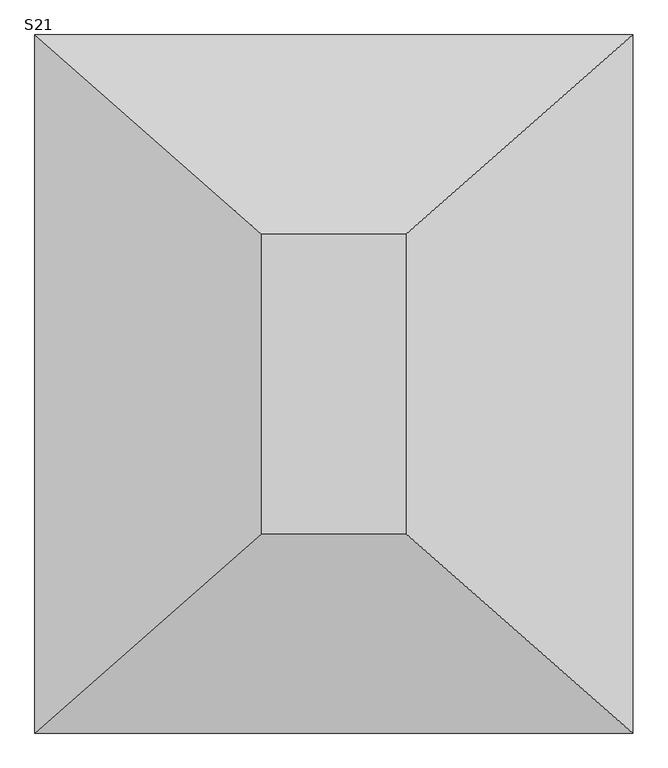
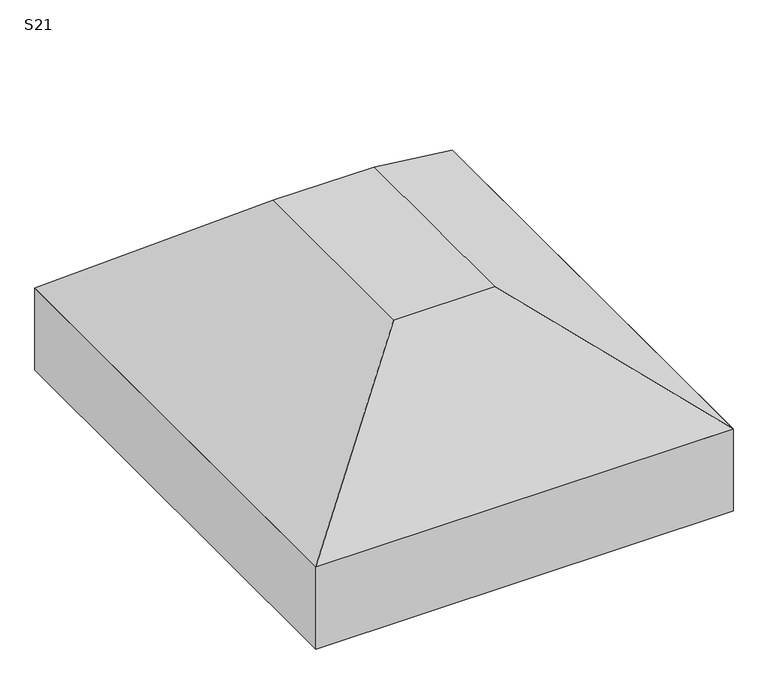
"""IFC4 building model written with IfcOpenShell, lengths in millimetres: fastener geometry, TQS - Sapata : S21."""

from ifc_helpers import new_model, si_unit, frame, origin, place, context, project, spatial, polyline, outline, extrude, faceted_brep, source, transform, mapped, element, save


def s21_dbbb6426(model_context):
    return source(origin(), model_context, "Body", "SolidModel", [
        faceted_brep([(-55.0, 100.0, 0.0), (-345.0, 100.0, 0.0), (-345.0, -500.0, 0.0), (-55.0, -500.0, 0.0), (400.0, 500.0, -350.0), (400.0, -900.0, -350.0), (-800.0, -900.0, -350.0), (-800.0, 500.0, -350.0)], [[[0, 1, 2, 3]], [[4, 5, 6, 7]], [[4, 7, 1, 0]], [[7, 6, 2, 1]], [[6, 5, 3, 2]], [[5, 4, 0, 3]]]),
        extrude(outline(polyline([(400.0, 500.0), (400.0, -900.0), (-800.0, -900.0), (-800.0, 500.0), (400.0, 500.0)])), frame((0.0, 0.0, -600.0), z_axis=(0.0, 0.0, 1.0), x_axis=(1.0, 0.0, 0.0)), (0.0, 0.0, 1.0), 250.0),
    ])


if __name__ == "__main__":
    model = new_model("IFC4")
    model_context = context("Model", 3, world=origin())
    ifc_project = project(units=[si_unit("LENGTHUNIT", "METRE", prefix="MILLI")], contexts=[model_context])
    site = spatial("IfcSite", under=ifc_project)
    building = spatial("IfcBuilding", under=site)
    placement = place(None, origin())
    s21_shape = s21_dbbb6426(model_context)
    element("IfcFastener", 1, ObjectType="TQS - Sapata : S21", at=placement, inside=building, context=model_context, shape_type="MappedRepresentation", body=[
        mapped(s21_shape, transform((0.0, 0.0, 0.0), x_axis=(1.0, 0.0, 0.0), y_axis=(0.0, 1.0, 0.0), z_axis=(0.0, 0.0, 1.0))),
    ])
    save(model, "model.ifc")

# Revit data of these elements
# Type "TQS - Sapata : S21"
#   TY = 0.60 m
#   TX = 0.29 m
#   HS = 0.60 m
#   H0 = 0.25 m
#   EXCYABS = 0.70 m
#   EXCY = 0.00 m
#   EXCXABS = 0.60 m
#   EXCX = 0.00 m
#   DIMY = 1.40 m
#   DIMX = 1.20 m
#   Material estrutural = Concreto - Concreto concretado no local
#   Width = 0
#   Length = 0
# Element 1 (IfcFastener, "TQS - Sapata : S21")
#   Materials on its faces: "Concreto - Concreto concretado no local"
# Materials
#   "Concreto - Concreto concretado no local": class "Concreto", colour RGB 192 192 192, transparency 0
